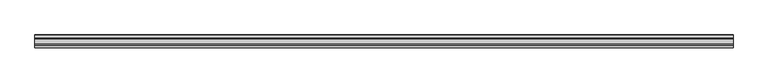
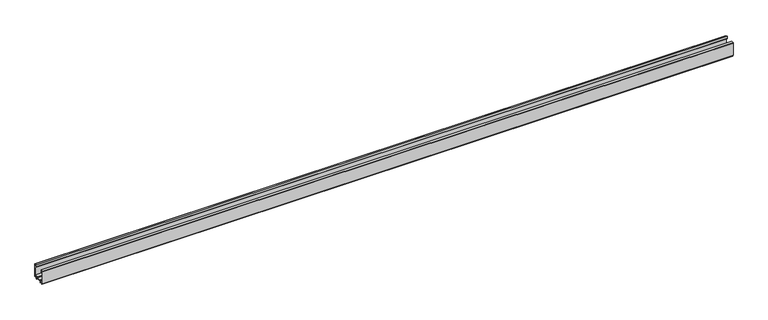
"""IFC4 building model written with IfcOpenShell, lengths in millimetres: proxy geometry, Generic Models 3:Generic Models 2:312240:Generic Models 2:312240 : Generic Models 3:Generic Models 2:312240:2 : Generic Models 3:Generic Models 2:312240:Generic Models 2:312240 : Generic Models 3:Generic Models 2:312240:300533."""

from ifc_helpers import new_model, si_unit, frame, origin, place, context, project, spatial, polyline, outline, extrude, source, transform, mapped, element, save


def generic_models_8b8b68aa(model_context):
    return source(origin(), model_context, "Body", "SweptSolid", [
        extrude(outline(polyline([(-536498.4587882, 8598.2706664), (-536497.5993089, 8598.7472945), (-536497.5993089, 8599.7980816), (-536507.5008029, 8601.2125807), (-536507.5008029, 8602.5847295), (-536495.3462744, 8602.5847295), (-536495.3462744, 8647.111807), (-536497.6585993, 8647.111807), (-536497.6585993, 8651.3807146), (-536495.8798878, 8656.242526), (-536497.6585993, 8656.5389779), (-536497.6585993, 8659.6813682), (-536492.2038841, 8659.6813682), (-536492.2038841, 8595.1734317), (-536495.3462744, 8595.1734317), (-536495.3462744, 8597.4857566), (-536496.7541511, 8597.4857566), (-536497.7674778, 8596.8270942), (-536498.5080328, 8597.3207976), (-536498.4587882, 8598.2706664)])), frame((592374.6787989, 0.0, 0.0), z_axis=(1.0, 0.0, 0.0), x_axis=(0.0, 1.0, 0.0)), (0.0, 0.0, 1.0), 3412.7573656),
        extrude(outline(polyline([(-536493.8163228, 8660.9177011), (-536493.8163228, 8659.8790879), (-536497.9491849, 8659.8790879), (-536497.9491849, 8656.1128501), (-536496.407148, 8655.855844), (-536497.9491849, 8651.6409432), (-536497.9491849, 8647.111807), (-536499.1544889, 8647.111807), (-536505.2477683, 8652.3604735), (-536505.2477683, 8663.9660865), (-536493.8163228, 8660.9177011)])), frame((592374.6787989, 0.0, 0.0), z_axis=(1.0, 0.0, 0.0), x_axis=(0.0, 1.0, 0.0)), (0.0, 0.0, 1.0), 3412.7573656),
        extrude(outline(polyline([(-536553.1543976, 8647.8232916), (-536553.1543976, 8604.8970545), (-536537.0867039, 8604.8970545), (-536537.0867039, 8598.0193701), (-536511.1768066, 8598.0193701), (-536511.1768066, 8604.8970545), (-536495.7020167, 8604.8970545), (-536495.7020167, 8603.3555045), (-536509.1609336, 8603.3555045), (-536509.1609336, 8598.0193701), (-536505.4256395, 8598.0193701), (-536504.121251, 8596.7149816), (-536497.302857, 8596.7149816), (-536496.3542109, 8597.3671759), (-536495.5241455, 8596.8335624), (-536495.5241455, 8595.4698836), (-536504.121251, 8595.4698836), (-536504.121251, 8589.185103), (-536506.1371241, 8589.185103), (-536506.1371241, 8595.4698836), (-536537.2052846, 8595.4698836), (-536537.2052846, 8589.185103), (-536539.2211577, 8589.185103), (-536539.2211577, 8595.4698836), (-536550.1305881, 8595.4698836), (-536550.1305881, 8589.185103), (-536552.1464611, 8589.185103), (-536552.1464611, 8595.4698836), (-536555.7038841, 8595.4698836), (-536555.7038841, 8657.8971156), (-536548.5890382, 8658.4955605), (-536548.5890382, 8653.455878), (-536549.8934266, 8653.2331775), (-536549.8934266, 8655.2664011), (-536551.4840848, 8655.2664011), (-536552.3695065, 8653.367608), (-536552.3695065, 8651.086189), (-536551.3756861, 8649.3648416), (-536549.8934266, 8649.3648416), (-536549.8934266, 8651.1731587), (-536548.5890382, 8649.8688863), (-536548.5890382, 8647.8232916), (-536553.1543976, 8647.8232916)]), holes=[polyline([(-536552.5614938, 8597.6043374), (-536539.2211577, 8597.6043374), (-536539.2211577, 8603.3555045), (-536552.5614938, 8603.3555045), (-536552.5614938, 8597.6043374)])]), frame((592374.6787989, 0.0, 0.0), z_axis=(1.0, 0.0, 0.0), x_axis=(0.0, 1.0, 0.0)), (0.0, 0.0, 1.0), 3412.7573656),
        extrude(outline(polyline([(-536545.2477683, 8662.4759105), (-536545.2477683, 8647.8232916), (-536548.2821927, 8647.8232916), (-536548.2821927, 8650.0515316), (-536550.1206041, 8651.889943), (-536550.1206041, 8649.6355548), (-536551.209791, 8649.6355548), (-536552.0702393, 8651.125895), (-536552.0702393, 8653.2061935), (-536551.2301937, 8655.0076771), (-536550.2058448, 8655.0076771), (-536550.2058448, 8652.9694138), (-536548.2821927, 8653.2978422), (-536548.2821927, 8658.7381419), (-536555.2064077, 8658.1557313), (-536555.2064077, 8660.2571463), (-536545.2477683, 8662.4759105)])), frame((592374.6787989, 0.0, 0.0), z_axis=(1.0, 0.0, 0.0), x_axis=(0.0, 1.0, 0.0)), (0.0, 0.0, 1.0), 3412.7573656),
    ])


if __name__ == "__main__":
    model = new_model("IFC4")
    model_context = context("Model", 3, world=origin())
    ifc_project = project(units=[si_unit("LENGTHUNIT", "METRE", prefix="MILLI")], contexts=[model_context])
    site = spatial("IfcSite", under=ifc_project)
    building = spatial("IfcBuilding", under=site)
    placement = place(None, origin())
    generic_models_shape = generic_models_8b8b68aa(model_context)
    element("IfcBuildingElementProxy", 1, Name="Generic Models 3:Generic Models 2:312240:Generic Models 2:312240 : Generic Models 3:Generic Models 2:312240:2 : Generic Models 3:Generic Models 2:312240:Generic Models 2:312240 : Generic Models 3:Generic Models 2:312240:300533", ObjectType="Generic Models 3:Generic Models 2:312240:Generic Models 2:312240 : Generic Models 3:Generic Models 2:312240:2 : Generic Models 3:Generic Models 2:312240:Generic Models 2:312240 : Generic Models 3:Generic Models 2:312240:300533", at=placement, inside=building, context=model_context, shape_type="MappedRepresentation", body=[
        mapped(generic_models_shape, transform((0.0, 0.0, 0.0), x_axis=(1.0, 0.0, 0.0), y_axis=(0.0, 1.0, 0.0), z_axis=(0.0, 0.0, 1.0))),
    ])
    save(model, "model.ifc")

# Revit data of these elements
# Type "Generic Models 3:Generic Models 2:312240:Generic Models 2:312240 : Generic Models 3:Generic Models 2:312240:2 : Generic Models 3:Generic Models 2:312240:Generic Models 2:312240 : Generic Models 3:Generic Models 2:312240:300533"
#   NameOverride = "Generic Models 3:Generic Models 2:312240:Generic Models 2:312240 : Generic Models 3:Generic Models 2:312240:300533"
#   ObjectTypeOverride = "Generic Models 2:312240 : Generic Models 3:Generic Models 2:312240"
#   Reference = "Generic Models 2"
#   Tag = "300533"
# Element 1 (IfcBuildingElementProxy, "Generic Models 3:Generic Models 2:312240:Generic Models 2:312240 : Generic Models 3:Generic Models 2:312240:2 : Generic Models 3:Generic Models 2:312240:Generic Models 2:312240 : Generic Models 3:Generic Models 2:312240:300533")
#   Materials on its faces: "THERMAL BROKEN ALUMINUM STOREFRONT FOR POLYCARBONATE"
# Materials
#   "THERMAL BROKEN ALUMINUM STOREFRONT FOR POLYCARBONATE": class "Unassigned", colour RGB 244 244 244, transparency 0, Keynote = "M07611300.01", Cost = 0
